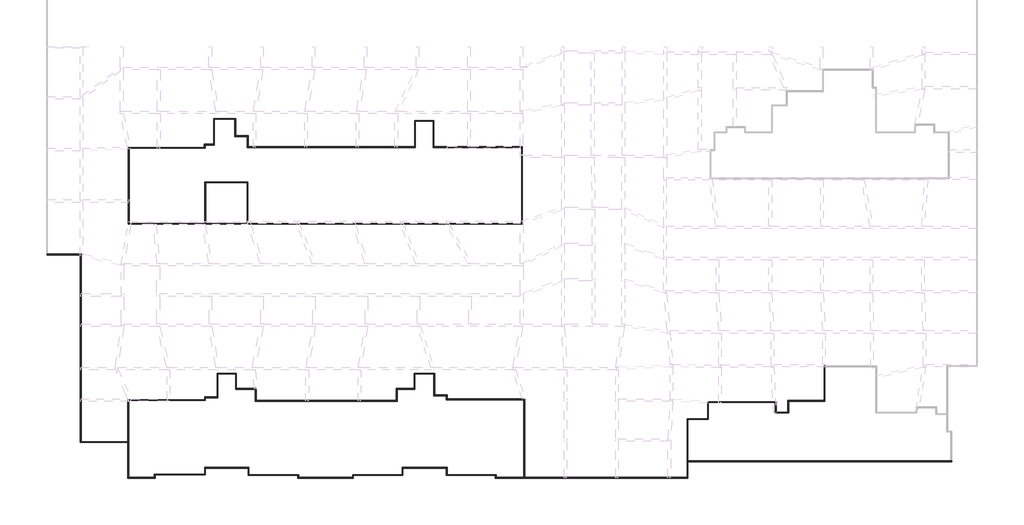
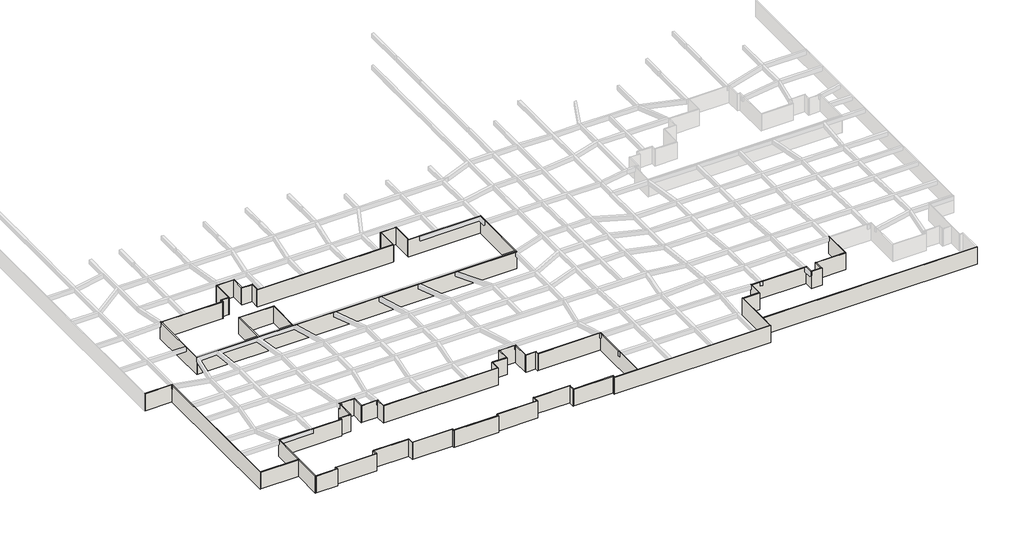
# One storey, part 1 of 45: 68 walls.
# Revit data of these elements (continued)
# Room, not placed, phase "新构造", upper offset 0 mm, lower offset 0 mm (continued)
#   Name = "客餐厅"
# Room, not placed, phase "新构造", upper offset 0 mm, lower offset 0 mm
#   Number = "2"
#   Name = "阳台"
# Room, not placed, phase "新构造", upper offset 0 mm, lower offset 0 mm
#   Number = "3"
#   Name = "次卧"
# Room, not placed, phase "新构造", upper offset 0 mm, lower offset 0 mm
#   Number = "4"
#   Name = "厨房"
# Area at (1120.278, 64973.048) mm, upper offset 0 mm, lower offset 0 mm
#   Number = "108"
#   Name = "main_building"
# Room, not placed, phase "新构造", upper offset 0 mm, lower offset 0 mm
#   Number = "5"
#   Name = "卫生间"
# Room, not placed, phase "新构造", upper offset 0 mm, lower offset 0 mm
#   Number = "6"
#   Name = "次卧"
# Room, not placed, phase "新构造", upper offset 0 mm, lower offset 0 mm
#   Number = "7"
#   Name = "主卧"
# Area, not placed, upper offset 0 mm, lower offset 0 mm
#   Number = "60"
#   Name = "fire_compart"
# Area, not placed, upper offset 0 mm, lower offset 0 mm
#   Number = "23"
#   Name = "main_building"
# Area at (-138124.742, 170633.157) mm, upper offset 0 mm, lower offset 0 mm
#   Number = "124"
#   Name = "fire_compart"
# Area, not placed, upper offset 0 mm, lower offset 0 mm
#   Number = "36"
#   Name = "main_building"
# Area, not placed, upper offset 0 mm, lower offset 0 mm
#   Number = "37"
#   Name = "main_building"
# Area, not placed, upper offset 0 mm, lower offset 0 mm
#   Number = "38"
#   Name = "main_building"
# Area, not placed, upper offset 0 mm, lower offset 0 mm
#   Number = "39"
#   Name = "main_building"
# Area, not placed, upper offset 0 mm, lower offset 0 mm
#   Number = "40"
#   Name = "main_building"
# Area, not placed, upper offset 0 mm, lower offset 0 mm
#   Number = "64"
#   Name = "fire_compart"
# Area, not placed, upper offset 0 mm, lower offset 0 mm
#   Number = "61"
#   Name = "fire_compart"
# Area, not placed, upper offset 0 mm, lower offset 0 mm
#   Number = "65"
#   Name = "main_building"
# Area at (-41970.473, 129859.608) mm, upper offset 0 mm, lower offset 0 mm
#   Number = "104"
#   Name = "main_building"
# Area, not placed, upper offset 0 mm, lower offset 0 mm
#   Number = "62"
#   Name = "fire_compart"
# Area at (-97187.783, 170360.042) mm, upper offset 0 mm, lower offset 0 mm
#   Number = "125"
#   Name = "fire_compart"
# Area, not placed, upper offset 0 mm, lower offset 0 mm
#   Number = "63"
#   Name = "fire_compart"
# Area, not placed, upper offset 0 mm, lower offset 0 mm
#   Number = "66"
#   Name = "main_building"
# Area at (-80006.909, 155700.134) mm, upper offset 0 mm, lower offset 0 mm
#   Number = "126"
#   Name = "fire_compart"
# Area, not placed, upper offset 0 mm, lower offset 0 mm
#   Number = "83"
#   Name = "fire_compart"
# Area, not placed, upper offset 0 mm, lower offset 0 mm
#   Number = "84"
#   Name = "main_building"
# Area, not placed, upper offset 0 mm, lower offset 0 mm
#   Number = "7"
#   Name = "fire_compart_5"
# Area at (-25400.176, 169838.842) mm, upper offset 0 mm, lower offset 0 mm
#   Number = "127"
#   Name = "fire_compart"
# Area at (35437.967, 169696.342) mm, upper offset 0 mm, lower offset 0 mm
#   Number = "128"
#   Name = "fire_compart"
# Area at (-3487.047, 206795.2) mm, upper offset 0 mm, lower offset 0 mm
#   Number = "129"
#   Name = "fire_compart"
# Area at (31234.14, 202640.995) mm, upper offset 0 mm, lower offset 0 mm
#   Number = "130"
#   Name = "fire_compart"
# Area at (-130444.27, 32041.624) mm, upper offset 0 mm, lower offset 0 mm
#   Number = "109"
#   Name = "main_building"
# Area, not placed, upper offset 0 mm, lower offset 0 mm
#   Number = "67"
#   Name = "fire_compart"
# Area at (42644.216, -30321.192) mm, upper offset 0 mm, lower offset 0 mm
#   Number = "112"
#   Name = "main_building"
# Area at (-146298.184, 112981.21) mm, upper offset 0 mm, lower offset 0 mm
#   Number = "131"
#   Name = "fire_compart"
# Area, not placed, upper offset 0 mm, lower offset 0 mm
#   Number = "68"
#   Name = "fire_compart"
# Area at (-121673.284, 111921.061) mm, upper offset 0 mm, lower offset 0 mm
#   Number = "132"
#   Name = "fire_compart"
# Area, not placed, upper offset 0 mm, lower offset 0 mm
#   Number = "1"
#   Name = "面积"
# Area, not placed, upper offset 0 mm, lower offset 0 mm
#   Number = "2"
#   Name = "防火区域1"
# Area at (-30897.039, 105171.206) mm, upper offset 0 mm, lower offset 0 mm
#   Number = "133"
#   Name = "fire_compart"
# Area at (11755.406, -2112.84) mm, upper offset 0 mm, lower offset 0 mm
#   Number = "144"
#   Name = "fire_compart"
# Area at (33484.528, 100314.6) mm, upper offset 0 mm, lower offset 0 mm
#   Number = "134"
#   Name = "fire_compart"
# Area, not placed, upper offset 0 mm, lower offset 0 mm
#   Number = "25"
#   Name = "fire_compart"
# Area, not placed, upper offset 0 mm, lower offset 0 mm
#   Number = "26"
#   Name = "fire_compart"
# Area, not placed, upper offset 0 mm, lower offset 0 mm
#   Number = "27"
#   Name = "fire_compart"
# Area, not placed, upper offset 0 mm, lower offset 0 mm
#   Number = "69"
#   Name = "fire_compart"
# Area at (39447.053, 124280.17) mm, upper offset 0 mm, lower offset 0 mm
#   Number = "105"
#   Name = "main_building"
# Area at (-7936.471, -47261.404) mm, upper offset 0 mm, lower offset 0 mm
#   Number = "113"
#   Name = "main_building"
# Area at (-124565.318, 62952.996) mm, upper offset 0 mm, lower offset 0 mm
#   Number = "135"
#   Name = "fire_compart"
# Area, not placed, upper offset 0 mm, lower offset 0 mm
#   Number = "85"
#   Name = "fire_compart"
# Area, not placed, upper offset 0 mm, lower offset 0 mm
#   Number = "86"
#   Name = "main_building"
# Area, not placed, upper offset 0 mm, lower offset 0 mm
#   Number = "87"
#   Name = "main_building"
# Area at (-48193.172, 45179.632) mm, upper offset 0 mm, lower offset 0 mm
#   Number = "136"
#   Name = "fire_compart"
# Room, not placed, phase "新构造", upper offset 0 mm, lower offset 0 mm
#   Number = "8"
#   Name = "客餐厅"
# Area, not placed, upper offset 0 mm, lower offset 0 mm
#   Number = "70"
#   Name = "main_building"
# Area at (54232.634, -90977.069) mm, upper offset 0 mm, lower offset 0 mm
#   Number = "114"
#   Name = "main_building"
# Area, not placed, upper offset 0 mm, lower offset 0 mm
#   Number = "8"
#   Name = "fire_compart_6"
# Area at (6775.356, 45964.064) mm, upper offset 0 mm, lower offset 0 mm
#   Number = "137"
#   Name = "fire_compart"
# Area at (-103298.192, 4854.348) mm, upper offset 0 mm, lower offset 0 mm
#   Number = "138"
#   Name = "fire_compart"
# Area, not placed, upper offset 0 mm, lower offset 0 mm
#   Number = "3"
#   Name = "fire_compart_1"
# Area at (-123001.657, -42543.294) mm, upper offset 0 mm, lower offset 0 mm
#   Number = "139"
#   Name = "fire_compart"
# Area, not placed, upper offset 0 mm, lower offset 0 mm
#   Number = "71"
#   Name = "fire_compart"
# Room, not placed, phase "新构造", upper offset 0 mm, lower offset 0 mm
#   Number = "11"
#   Name = "房间"
# Area at (-118996.669, -120161.362) mm, upper offset 0 mm, lower offset 0 mm
#   Number = "140"
#   Name = "fire_compart"
# Area at (55095.998, 72501.978) mm, upper offset 0 mm, lower offset 0 mm
#   Number = "106"
#   Name = "main_building"
# Room, not placed, phase "新构造", upper offset 0 mm, lower offset 0 mm
#   Number = "12"
#   Name = "房间"
# Area at (53847.098, 13133.356) mm, upper offset 0 mm, lower offset 0 mm
#   Number = "110"
#   Name = "main_building"
# Area at (-32471.188, -169087.975) mm, upper offset 0 mm, lower offset 0 mm
#   Number = "141"
#   Name = "fire_compart"
# Area at (-136920.698, 200560.172) mm, upper offset 0 mm, lower offset 0 mm
#   Number = "100"
#   Name = "main_building"
# Room, not placed, phase "新构造", upper offset 0 mm, lower offset 0 mm
#   Number = "13"
#   Name = "房间"
# Room, not placed, phase "新构造", upper offset 0 mm, lower offset 0 mm
#   Number = "14"
#   Name = "房间"
# Area, not placed, upper offset 0 mm, lower offset 0 mm
#   Number = "72"
#   Name = "main_building"
# Room, not placed, phase "新构造", upper offset 0 mm, lower offset 0 mm
#   Number = "15"
#   Name = "房间"
# Area, not placed, upper offset 0 mm, lower offset 0 mm
#   Number = "88"
#   Name = "fire_compart"
# Room, not placed, phase "新构造", upper offset 0 mm, lower offset 0 mm
#   Number = "16"
#   Name = "房间"
# Area, not placed, upper offset 0 mm, lower offset 0 mm
#   Number = "28"
#   Name = "面积"
# Area, not placed, upper offset 0 mm, lower offset 0 mm
#   Number = "73"
#   Name = "fire_compart"
# Area at (-34365.786, -184880.66) mm, upper offset 0 mm, lower offset 0 mm
#   Number = "116"
#   Name = "main_building"
# Area at (-30701.012, 193486.781) mm, upper offset 0 mm, lower offset 0 mm
#   Number = "101"
#   Name = "main_building"
# Room, not placed, phase "新构造", upper offset 0 mm, lower offset 0 mm
#   Number = "17"
#   Name = "房间"
# Area, not placed, upper offset 0 mm, lower offset 0 mm
#   Number = "30"
#   Name = "main_building"
# Area at (-56072.822, -2322.739) mm, upper offset 0 mm, lower offset 0 mm
#   Number = "143"
#   Name = "fire_compart"
# Area, not placed, upper offset 0 mm, lower offset 0 mm
#   Number = "89"
#   Name = "main_building"
# Area, not placed, upper offset 0 mm, lower offset 0 mm
#   Number = "75"
#   Name = "main_building"
# Area at (-37353.761, 13292.404) mm, upper offset 0 mm, lower offset 0 mm
#   Number = "111"
#   Name = "main_building"
# Area, not placed, upper offset 0 mm, lower offset 0 mm
#   Number = "90"
#   Name = "fire_compart"
# Area, not placed, upper offset 0 mm, lower offset 0 mm
#   Number = "76"
#   Name = "main_building"
# Area at (40608.048, -69765.274) mm, upper offset 0 mm, lower offset 0 mm
#   Number = "145"
#   Name = "fire_compart"
# Area at (-41821.749, -71305.293) mm, upper offset 0 mm, lower offset 0 mm
#   Number = "146"
#   Name = "fire_compart"
# Area at (-2956.6, -87290.297) mm, upper offset 0 mm, lower offset 0 mm
#   Number = "147"
#   Name = "fire_compart"
# Area at (-124032.628, -146786.551) mm, upper offset 0 mm, lower offset 0 mm
#   Number = "117"
#   Name = "main_building"
# Area, not placed, upper offset 0 mm, lower offset 0 mm
#   Number = "4"
#   Name = "fire_compart_2"
# Area, not placed, upper offset 0 mm, lower offset 0 mm
#   Number = "77"
#   Name = "main_building"
# Area, not placed, upper offset 0 mm, lower offset 0 mm
#   Number = "78"
#   Name = "main_building"
# Area, not placed, upper offset 0 mm, lower offset 0 mm
#   Number = "79"
#   Name = "main_building"
# Area, not placed, upper offset 0 mm, lower offset 0 mm
#   Number = "29"
#   Name = "main_building"
